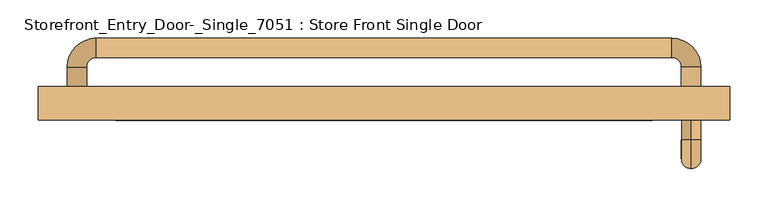
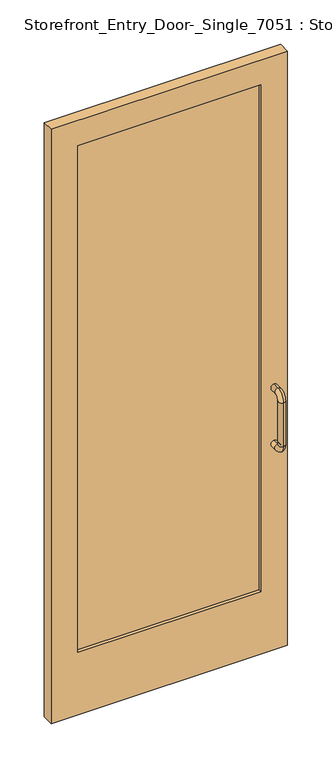
"""IFC4 building model written with IfcOpenShell, lengths in millimetres: door geometry, Storefront_Entry_Door-_Single_7051 : Store Front Single Door."""

from ifc_helpers import new_model, si_unit, point, frame, origin, place, context, project, spatial, polyline, circle_curve, ellipse_curve, trimmed, outline, extrude, source, transform, mapped, element, save
from ifc_brep_helpers import plane_surface, cylinder_surface, revolved_surface, advanced_brep


def storefront_entry_door_single_7051_store_front_single_door_ff742114(model_context):
    return source(origin(), model_context, "Body", "SolidModel", [
        advanced_brep(
        [(402.7714285, -50.8, 1054.1), (402.7714285, -50.8, 1079.5), (402.7714285, -76.2, 1079.5), (402.7714285, -76.2, 1054.1), (402.7714285, -114.3, 1041.4), (402.7714285, -88.9, 1041.4), (402.7714285, -114.3, 863.6), (402.7714285, -88.9, 863.6), (402.7714285, -76.2, 825.5), (402.7714285, -76.2, 850.9), (402.7714285, -50.8, 850.9), (402.7714285, -50.8, 825.5)],
        [
            (0, 1, circle_curve(frame((402.7714285, -50.8, 1066.8), z_axis=(0.0, 1.0, 0.0), x_axis=(0.0, 0.0, 1.0)), 12.7)),
            (1, 0, circle_curve(frame((402.7714285, -50.8, 1066.8), z_axis=(0.0, 1.0, 0.0), x_axis=(0.0, 0.0, 1.0)), 12.7)),
            (1, 2),
            (2, 3, circle_curve(frame((402.7714285, -76.2, 1066.8), z_axis=(0.0, 1.0, 0.0), x_axis=(0.0, 0.0, 1.0)), 12.7)),
            (3, 0),
            (3, 2, circle_curve(frame((402.7714285, -76.2, 1066.8), z_axis=(0.0, 1.0, 0.0), x_axis=(0.0, 0.0, 1.0)), 12.7)),
            (4, 5, circle_curve(frame((402.7714285, -101.6, 1041.4), z_axis=(0.0, 0.0, 1.0), x_axis=(0.0, -1.0, 0.0)), 12.7)),
            (5, 3, circle_curve(frame((402.7714285, -76.2, 1041.4), z_axis=(-1.0, 0.0, 0.0), x_axis=(0.0, 0.0, 1.0)), 12.7)),
            (2, 4, circle_curve(frame((402.7714285, -76.2, 1041.4), z_axis=(1.0, 0.0, 0.0), x_axis=(0.0, 0.0, 1.0)), 38.1)),
            (5, 4, circle_curve(frame((402.7714285, -101.6, 1041.4), z_axis=(0.0, 0.0, 1.0), x_axis=(0.0, -1.0, 0.0)), 12.7)),
            (4, 6),
            (6, 7, circle_curve(frame((402.7714285, -101.6, 863.6), z_axis=(0.0, 0.0, 1.0), x_axis=(0.0, -1.0, 0.0)), 12.7)),
            (7, 5),
            (7, 6, circle_curve(frame((402.7714285, -101.6, 863.6), z_axis=(0.0, 0.0, 1.0), x_axis=(0.0, -1.0, 0.0)), 12.7)),
            (8, 9, circle_curve(frame((402.7714285, -76.2, 838.2), z_axis=(0.0, -1.0, 0.0), x_axis=(0.0, 0.0, -1.0)), 12.7)),
            (9, 7, circle_curve(frame((402.7714285, -76.2, 863.6), z_axis=(-1.0, 0.0, 0.0), x_axis=(0.0, -1.0, 0.0)), 12.7)),
            (6, 8, circle_curve(frame((402.7714285, -76.2, 863.6), z_axis=(1.0, 0.0, 0.0), x_axis=(0.0, -1.0, 0.0)), 38.1)),
            (9, 8, circle_curve(frame((402.7714285, -76.2, 838.2), z_axis=(0.0, -1.0, 0.0), x_axis=(0.0, 0.0, -1.0)), 12.7)),
            (10, 11, circle_curve(frame((402.7714285, -50.8, 838.2), z_axis=(0.0, 1.0, 0.0), x_axis=(0.0, 0.0, -1.0)), 12.7)),
            (11, 10, circle_curve(frame((402.7714285, -50.8, 838.2), z_axis=(0.0, 1.0, 0.0), x_axis=(0.0, 0.0, -1.0)), 12.7)),
            (8, 11),
            (10, 9),
        ],
        [
            plane_surface(frame((402.7714285, -50.8, 1066.8), z_axis=(0.0, 1.0, 0.0), x_axis=(1.0, 0.0, 0.0))),
            cylinder_surface(frame((402.7714285, -50.8, 1066.8), z_axis=(0.0, 1.0, 0.0), x_axis=(0.0, 0.0, 1.0)), 12.7),
            revolved_surface(trimmed(ellipse_curve(frame((402.7714285, -76.2, 1066.8), z_axis=(0.0, -1.0, 0.0), x_axis=(0.0, 0.0, 1.0)), 12.7, 12.7), [point((402.7714285, -76.2, 1054.1))], [point((402.7714285, -76.2, 1079.5))], True, "CARTESIAN"), (402.7714285, -76.2, 1041.4), (-1.0, 0.0, 0.0)),
            revolved_surface(trimmed(ellipse_curve(frame((402.7714285, -76.2, 1066.8), z_axis=(0.0, -1.0, 0.0), x_axis=(0.0, 0.0, 1.0)), 12.7, 12.7), [point((402.7714285, -76.2, 1079.5))], [point((402.7714285, -76.2, 1054.1))], True, "CARTESIAN"), (402.7714285, -76.2, 1041.4), (-1.0, 0.0, 0.0)),
            cylinder_surface(frame((402.7714285, -101.6, 1041.4), z_axis=(0.0, 0.0, 1.0), x_axis=(0.0, -1.0, 0.0)), 12.7),
            revolved_surface(trimmed(ellipse_curve(frame((402.7714285, -101.6, 863.6), z_axis=(0.0, 0.0, -1.0), x_axis=(0.0, -1.0, 0.0)), 12.7, 12.7), [point((402.7714285, -88.9, 863.6))], [point((402.7714285, -114.3, 863.6))], True, "CARTESIAN"), (402.7714285, -76.2, 863.6), (-1.0, 0.0, 0.0)),
            revolved_surface(trimmed(ellipse_curve(frame((402.7714285, -101.6, 863.6), z_axis=(0.0, 0.0, -1.0), x_axis=(0.0, -1.0, 0.0)), 12.7, 12.7), [point((402.7714285, -114.3, 863.6))], [point((402.7714285, -88.9, 863.6))], True, "CARTESIAN"), (402.7714285, -76.2, 863.6), (-1.0, 0.0, 0.0)),
            plane_surface(frame((402.7714285, -50.8, 838.2), z_axis=(0.0, 1.0, 0.0), x_axis=(1.0, 0.0, 0.0))),
            cylinder_surface(frame((402.7714285, -76.2, 838.2), z_axis=(0.0, -1.0, 0.0), x_axis=(0.0, 0.0, -1.0)), 12.7),
        ],
        [
            (0, [[1, 2]]),
            (1, [[3, 4, 5, -2]]),
            (1, [[-5, 6, -3, -1]]),
            (2, [[7, 8, -4, 9]]),
            (3, [[10, -9, -6, -8]]),
            (4, [[11, 12, 13, -7]]),
            (4, [[-13, 14, -11, -10]]),
            (5, [[15, 16, -12, 17]]),
            (6, [[18, -17, -14, -16]]),
            (7, [[19, 20]]),
            (8, [[21, -19, 22, -15]]),
            (8, [[-22, -20, -21, -18]]),
        ],
    ),
        advanced_brep(
        [(390.0714285, -6.35, 1066.8), (415.4714285, -6.35, 1066.8), (415.4714285, 19.05, 1066.8), (390.0714285, 19.05, 1066.8), (377.3714285, 57.15, 1066.8), (377.3714285, 31.75, 1066.8), (-377.3714285, 57.15, 1066.8), (-377.3714285, 31.75, 1066.8), (-415.4714285, 19.05, 1066.8), (-390.0714285, 19.05, 1066.8), (-390.0714285, -6.35, 1066.8), (-415.4714285, -6.35, 1066.8)],
        [
            (0, 1, circle_curve(frame((402.7714285, -6.35, 1066.8), z_axis=(0.0, -1.0, 0.0), x_axis=(1.0, 0.0, 0.0)), 12.7)),
            (1, 0, circle_curve(frame((402.7714285, -6.35, 1066.8), z_axis=(0.0, -1.0, 0.0), x_axis=(1.0, 0.0, 0.0)), 12.7)),
            (1, 2),
            (2, 3, circle_curve(frame((402.7714285, 19.05, 1066.8), z_axis=(0.0, -1.0, 0.0), x_axis=(1.0, 0.0, 0.0)), 12.7)),
            (3, 0),
            (3, 2, circle_curve(frame((402.7714285, 19.05, 1066.8), z_axis=(0.0, -1.0, 0.0), x_axis=(1.0, 0.0, 0.0)), 12.7)),
            (4, 5, circle_curve(frame((377.3714285, 44.45, 1066.8), z_axis=(1.0, 0.0, 0.0), x_axis=(0.0, 1.0, 0.0)), 12.7)),
            (5, 3, circle_curve(frame((377.3714285, 19.05, 1066.8), z_axis=(0.0, 0.0, -1.0), x_axis=(1.0, 0.0, 0.0)), 12.7)),
            (2, 4, circle_curve(frame((377.3714285, 19.05, 1066.8), z_axis=(0.0, 0.0, 1.0), x_axis=(1.0, 0.0, 0.0)), 38.1)),
            (5, 4, circle_curve(frame((377.3714285, 44.45, 1066.8), z_axis=(1.0, 0.0, 0.0), x_axis=(0.0, 1.0, 0.0)), 12.7)),
            (4, 6),
            (6, 7, circle_curve(frame((-377.3714285, 44.45, 1066.8), z_axis=(1.0, 0.0, 0.0), x_axis=(0.0, 1.0, 0.0)), 12.7)),
            (7, 5),
            (7, 6, circle_curve(frame((-377.3714285, 44.45, 1066.8), z_axis=(1.0, 0.0, 0.0), x_axis=(0.0, 1.0, 0.0)), 12.7)),
            (8, 9, circle_curve(frame((-402.7714285, 19.05, 1066.8), z_axis=(0.0, 1.0, 0.0), x_axis=(-1.0, 0.0, 0.0)), 12.7)),
            (9, 7, circle_curve(frame((-377.3714285, 19.05, 1066.8), z_axis=(0.0, 0.0, -1.0), x_axis=(0.0, 1.0, 0.0)), 12.7)),
            (6, 8, circle_curve(frame((-377.3714285, 19.05, 1066.8), z_axis=(0.0, 0.0, 1.0), x_axis=(0.0, 1.0, 0.0)), 38.1)),
            (9, 8, circle_curve(frame((-402.7714285, 19.05, 1066.8), z_axis=(0.0, 1.0, 0.0), x_axis=(-1.0, 0.0, 0.0)), 12.7)),
            (10, 11, circle_curve(frame((-402.7714285, -6.35, 1066.8), z_axis=(0.0, -1.0, 0.0), x_axis=(-1.0, 0.0, 0.0)), 12.7)),
            (11, 10, circle_curve(frame((-402.7714285, -6.35, 1066.8), z_axis=(0.0, -1.0, 0.0), x_axis=(-1.0, 0.0, 0.0)), 12.7)),
            (8, 11),
            (10, 9),
        ],
        [
            plane_surface(frame((402.7714285, -6.35, 1066.8), z_axis=(0.0, -1.0, 0.0), x_axis=(0.0, 0.0, 1.0))),
            cylinder_surface(frame((402.7714285, -6.35, 1066.8), z_axis=(0.0, -1.0, 0.0), x_axis=(1.0, 0.0, 0.0)), 12.7),
            revolved_surface(trimmed(ellipse_curve(frame((402.7714285, 19.05, 1066.8), z_axis=(0.0, 1.0, 0.0), x_axis=(1.0, 0.0, 0.0)), 12.7, 12.7), [point((390.0714285, 19.05, 1066.8))], [point((415.4714285, 19.05, 1066.8))], True, "CARTESIAN"), (377.3714285, 19.05, 1066.8), (0.0, 0.0, -1.0)),
            revolved_surface(trimmed(ellipse_curve(frame((402.7714285, 19.05, 1066.8), z_axis=(0.0, 1.0, 0.0), x_axis=(1.0, 0.0, 0.0)), 12.7, 12.7), [point((415.4714285, 19.05, 1066.8))], [point((390.0714285, 19.05, 1066.8))], True, "CARTESIAN"), (377.3714285, 19.05, 1066.8), (0.0, 0.0, -1.0)),
            cylinder_surface(frame((377.3714285, 44.45, 1066.8), z_axis=(1.0, 0.0, 0.0), x_axis=(0.0, 1.0, 0.0)), 12.7),
            revolved_surface(trimmed(ellipse_curve(frame((-377.3714285, 44.45, 1066.8), z_axis=(-1.0, 0.0, 0.0), x_axis=(0.0, 1.0, 0.0)), 12.7, 12.7), [point((-377.3714285, 31.75, 1066.8))], [point((-377.3714285, 57.15, 1066.8))], True, "CARTESIAN"), (-377.3714285, 19.05, 1066.8), (0.0, 0.0, -1.0)),
            revolved_surface(trimmed(ellipse_curve(frame((-377.3714285, 44.45, 1066.8), z_axis=(-1.0, 0.0, 0.0), x_axis=(0.0, 1.0, 0.0)), 12.7, 12.7), [point((-377.3714285, 57.15, 1066.8))], [point((-377.3714285, 31.75, 1066.8))], True, "CARTESIAN"), (-377.3714285, 19.05, 1066.8), (0.0, 0.0, -1.0)),
            plane_surface(frame((-402.7714285, -6.35, 1066.8), z_axis=(0.0, -1.0, 0.0), x_axis=(0.0, 0.0, 1.0))),
            cylinder_surface(frame((-402.7714285, 19.05, 1066.8), z_axis=(0.0, 1.0, 0.0), x_axis=(-1.0, 0.0, 0.0)), 12.7),
        ],
        [
            (0, [[1, 2]]),
            (1, [[3, 4, 5, -2]]),
            (1, [[-5, 6, -3, -1]]),
            (2, [[7, 8, -4, 9]]),
            (3, [[10, -9, -6, -8]]),
            (4, [[11, 12, 13, -7]]),
            (4, [[-13, 14, -11, -10]]),
            (5, [[15, 16, -12, 17]]),
            (6, [[18, -17, -14, -16]]),
            (7, [[19, 20]]),
            (8, [[21, -19, 22, -15]]),
            (8, [[-22, -20, -21, -18]]),
        ],
    ),
        extrude(outline(polyline([(351.9714285, -19.05), (351.9714285, -38.1), (-351.9714285, -38.1), (-351.9714285, -19.05), (351.9714285, -19.05)])), frame((0.0, 0.0, 254.0), z_axis=(0.0, 0.0, 1.0), x_axis=(1.0, 0.0, 0.0)), (0.0, 0.0, 1.0), 2057.4),
        extrude(outline(polyline([(2413.0, 453.5714285), (2413.0, -453.5714285), (0.0, -453.5714285), (0.0, 453.5714285), (2413.0, 453.5714285)]), holes=[polyline([(2311.4, -351.9714285), (2311.4, 351.9714285), (254.0, 351.9714285), (254.0, -351.9714285), (2311.4, -351.9714285)])]), frame((0.0, -50.8, 0.0), z_axis=(0.0, 1.0, 0.0), x_axis=(0.0, 0.0, 1.0)), (0.0, 0.0, 1.0), 44.45),
    ])


if __name__ == "__main__":
    model = new_model("IFC4")
    model_context = context("Model", 3, world=origin())
    ifc_project = project(units=[si_unit("LENGTHUNIT", "METRE", prefix="MILLI")], contexts=[model_context])
    site = spatial("IfcSite", under=ifc_project)
    building = spatial("IfcBuilding", under=site)
    placement = place(None, origin())
    storefront_entry_door_single_7051_store_front_single_door_shape = storefront_entry_door_single_7051_store_front_single_door_ff742114(model_context)
    element("IfcDoor", 1, ObjectType="Storefront_Entry_Door-_Single_7051 : Store Front Single Door", at=placement, inside=building, context=model_context, shape_type="MappedRepresentation", body=[
        mapped(storefront_entry_door_single_7051_store_front_single_door_shape, transform((0.0, 0.0, 0.0), x_axis=(1.0, 0.0, 0.0), y_axis=(0.0, 1.0, 0.0), z_axis=(0.0, 0.0, 1.0))),
    ])
    save(model, "model.ifc")

# Revit data of these elements
# Type "Storefront_Entry_Door-_Single_7051 : Store Front Single Door"
#   Type Mark = "19"
#   Assembly Code = "B2030110"
#   Analytic Construction = "<None>"
#   Top Rail = 0' - 4"
#   Side Rail = 0' - 4"
#   Reporting Width [instance default] = 4' - 2"
#   Rail Height AFF = 3' - 6"
#   Offset = 0' - 2"
#   Door Width [instance default] = 4' - 2"
#   Bottom Rail Width = 0' - 10"
#   Material = Metal - Aluminum
#   Glazing Material = Glass
#   Function = (empty or 0)
# Element 1 (IfcDoor, "Storefront_Entry_Door-_Single_7051 : Store Front Single Door")
#   Reporting Width = 2' - 11.71429"
#   Door Width = 2' - 11.71429"
#   Materials on its faces: "Metal - Aluminum", "Glass"
# Materials
#   "Metal - Aluminum": class "Metal", colour RGB 247 247 247, transparency 0
#   "Glass": class "Glass", colour RGB 218 227 224, transparency 0.85, Description = "Soda Lime Glass", Cost = 0
